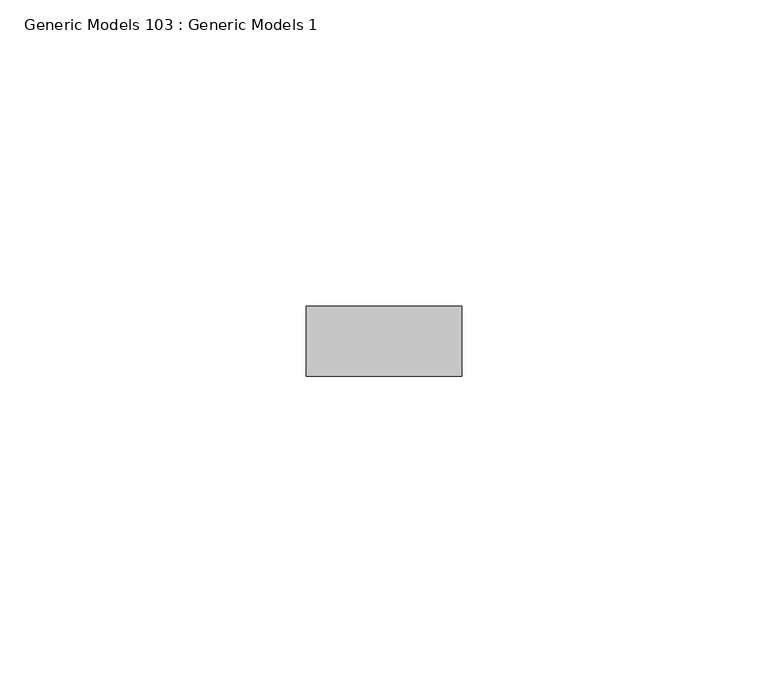
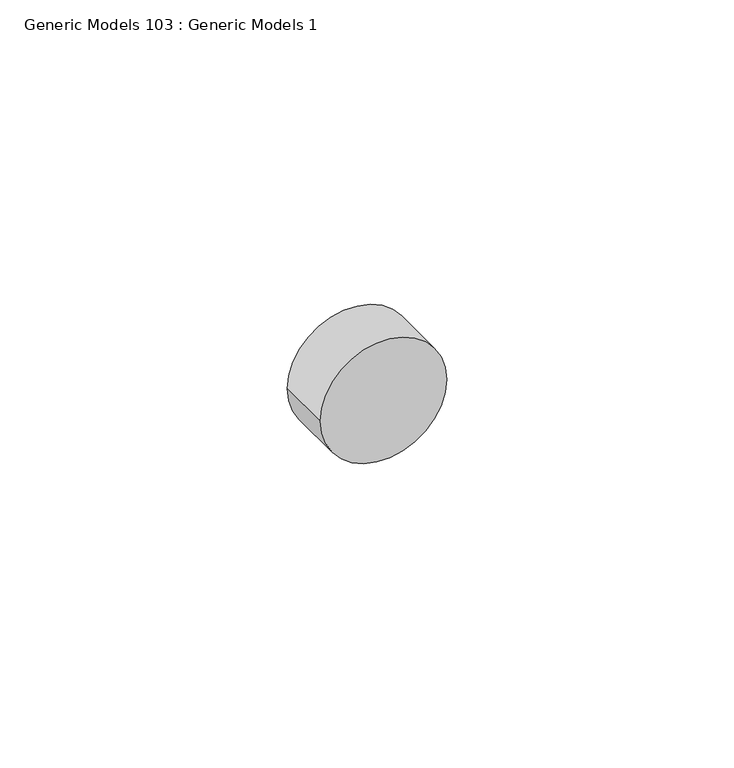
"""IFC4 building model written with IfcOpenShell, lengths in millimetres: proxy geometry, Generic Models 103 : Generic Models 1."""

from ifc_helpers import new_model, si_unit, point, frame, frame_2d, origin, place, context, project, spatial, circle_curve, trimmed, segment, composite_curve, outline, extrude, source, transform, mapped, element, save


def generic_models_103_generic_models_1_df1a5644(model_context):
    return source(origin(), model_context, "Body", "SweptSolid", [
        extrude(outline(composite_curve([segment(trimmed(circle_curve(frame_2d((37345.8776334, 5900.5346014)), 12.7), [point((37345.8776334, 5913.2346014))], [point((37345.8776334, 5887.8346014))], False, "CARTESIAN"), True, "CONTINUOUS"), segment(trimmed(circle_curve(frame_2d((37345.8776334, 5900.5346014)), 12.7), [point((37345.8776334, 5887.8346014))], [point((37345.8776334, 5913.2346014))], False, "CARTESIAN"), True, "CONTINUOUS")], self_intersect=False)), frame((0.0, 1836.9202358, 0.0), z_axis=(0.0, 1.0, 0.0), x_axis=(0.0, 0.0, 1.0)), (0.0, 0.0, 1.0), 11.4464372),
    ])


if __name__ == "__main__":
    model = new_model("IFC4")
    model_context = context("Model", 3, world=origin())
    ifc_project = project(units=[si_unit("LENGTHUNIT", "METRE", prefix="MILLI")], contexts=[model_context])
    site = spatial("IfcSite", under=ifc_project)
    building = spatial("IfcBuilding", under=site)
    placement = place(None, origin())
    generic_models_103_generic_models_1_shape = generic_models_103_generic_models_1_df1a5644(model_context)
    element("IfcBuildingElementProxy", 1, Name="Generic Models 103 : Generic Models 1", ObjectType="Generic Models 103 : Generic Models 1", at=placement, inside=building, context=model_context, shape_type="MappedRepresentation", body=[
        mapped(generic_models_103_generic_models_1_shape, transform((0.0, 0.0, 0.0), x_axis=(1.0, 0.0, 0.0), y_axis=(0.0, 1.0, 0.0), z_axis=(0.0, 0.0, 1.0))),
    ])
    save(model, "model.ifc")

# Revit data of these elements
# Element 1 (IfcBuildingElementProxy, "Generic Models 103 : Generic Models 1")
#   Materials on its faces: "S.S. LAG BOLT - SEE STRUCT. DWGS"
# Materials
#   "S.S. LAG BOLT - SEE STRUCT. DWGS": class "Generic", colour RGB 120 120 120, transparency 0, Cost = 0
